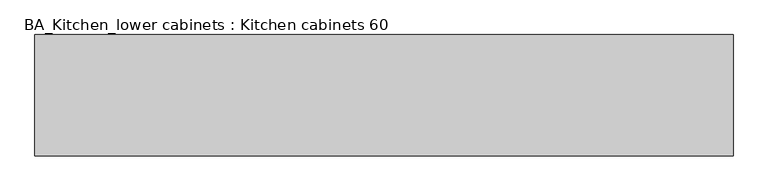
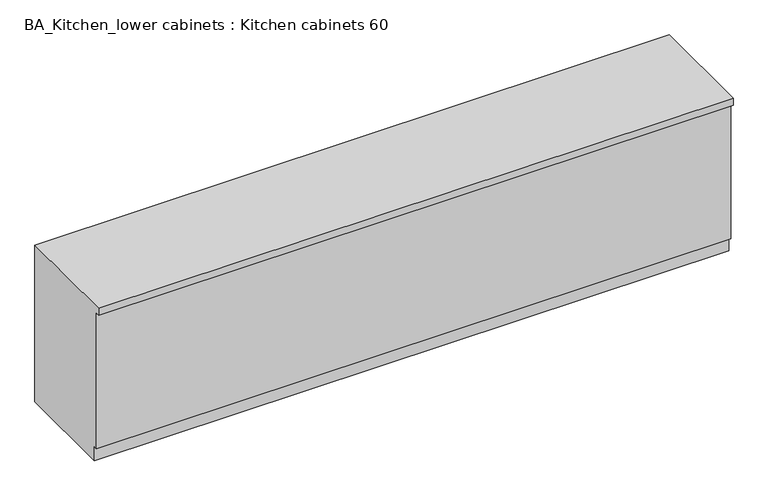
"""IFC4 building model written with IfcOpenShell, lengths in millimetres: furniture geometry, BA_Kitchen_lower cabinets : Kitchen cabinets 60."""

from ifc_helpers import new_model, si_unit, frame, origin, place, context, project, spatial, polyline, outline, extrude, source, transform, mapped, element, save


def ba_kitchen_lower_cabinets_kitchen_cabinets_60_4b58d319(model_context):
    return source(origin(), model_context, "Body", "SweptSolid", [
        extrude(outline(polyline([(-600.0, 900.0), (0.0, 900.0), (0.0, 0.0), (-560.0, 0.0), (-560.0, 80.0), (-580.0, 80.0), (-580.0, 860.0), (-600.0, 860.0), (-600.0, 900.0)])), frame((0.0, 0.0, 0.0), z_axis=(1.0, 0.0, 0.0), x_axis=(0.0, 1.0, 0.0)), (0.0, 0.0, 1.0), 3450.0),
    ])


if __name__ == "__main__":
    model = new_model("IFC4")
    model_context = context("Model", 3, world=origin())
    ifc_project = project(units=[si_unit("LENGTHUNIT", "METRE", prefix="MILLI")], contexts=[model_context])
    site = spatial("IfcSite", under=ifc_project)
    building = spatial("IfcBuilding", under=site)
    placement = place(None, origin())
    ba_kitchen_lower_cabinets_kitchen_cabinets_60_shape = ba_kitchen_lower_cabinets_kitchen_cabinets_60_4b58d319(model_context)
    element("IfcFurniture", 1, ObjectType="BA_Kitchen_lower cabinets : Kitchen cabinets 60", at=placement, inside=building, context=model_context, shape_type="MappedRepresentation", body=[
        mapped(ba_kitchen_lower_cabinets_kitchen_cabinets_60_shape, transform((0.0, 0.0, 0.0), x_axis=(1.0, 0.0, 0.0), y_axis=(0.0, 1.0, 0.0), z_axis=(0.0, 0.0, 1.0))),
    ])
    save(model, "model.ifc")

# Revit data of these elements
# Type "BA_Kitchen_lower cabinets : Kitchen cabinets 60"
#   built-in parameter 1001306 [instance default] = 4.85564 (stored number, unit not read)
#   Height [instance default] = 900 mm
#   Depth = 600 mm
#   Default Elevation = 0
# Element 1 (IfcFurniture, "BA_Kitchen_lower cabinets : Kitchen cabinets 60")
#   built-in parameter 1001306 = 11.3189 (stored number, unit not read)
#   Materials on its faces: "Default"
# Materials
#   "Default": class "Generic", colour RGB 255 255 255, transparency 0, Cost = 0
